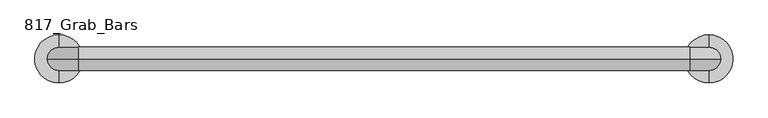
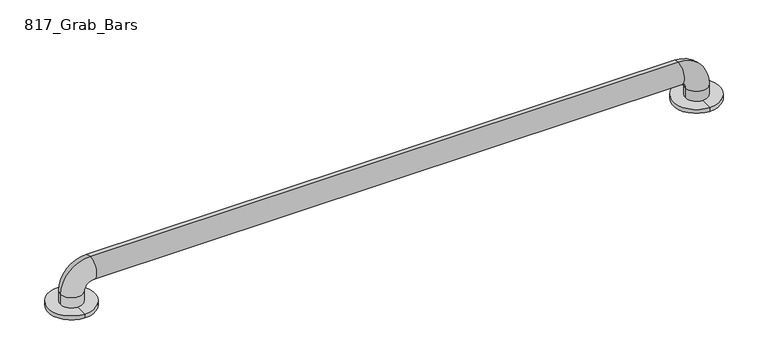
"""IFC4 building model written with IfcOpenShell, lengths in millimetres: proxy geometry, 817_Grab_Bars : 8170-001420."""

from ifc_helpers import new_model, si_unit, point, frame, origin, place, context, project, spatial, circle_curve, ellipse_curve, trimmed, source, transform, mapped, element, save
from ifc_brep_helpers import plane_surface, cylinder_surface, revolved_surface, advanced_brep


def proxy_817_grab_bars_e388bd4b(model_context):
    return source(origin(), model_context, "Body", "AdvancedBrep", [
        advanced_brep(
        [(-439.7375, -496.8875, 7.14375), (-439.7375, -576.2625, 7.14375), (-439.7375, -555.625, 7.14375), (-458.7875, -536.575, 7.14375), (-439.7375, -517.525, 7.14375), (-420.6875, -536.575, 7.14375), (-439.7375, -576.2625, 0.0), (-439.7375, -496.8875, 0.0), (-439.7375, -517.525, 0.0), (-439.7375, -536.575, 0.0), (-439.7375, -555.625, 0.0), (627.0625, -496.8875, 7.14375), (627.0625, -576.2625, 7.14375), (627.0625, -555.625, 7.14375), (608.0125, -536.575, 7.14375), (627.0625, -517.525, 7.14375), (646.1125, -536.575, 7.14375), (627.0625, -576.2625, 0.0), (627.0625, -496.8875, 0.0), (627.0625, -517.525, 0.0), (627.0625, -536.575, 0.0), (627.0625, -555.625, 0.0), (-458.7875, -536.575, 25.4), (-420.6875, -536.575, 25.4), (-407.9875, -536.575, 76.2), (-407.9875, -536.575, 38.1), (595.3125, -536.575, 76.2), (595.3125, -536.575, 38.1), (646.1125, -536.575, 25.4), (608.0125, -536.575, 25.4)],
        [
            (0, 1, circle_curve(frame((-439.7375, -536.575, 7.14375), z_axis=(0.0, 0.0, 1.0), x_axis=(0.0, 1.0, 0.0)), 39.6875)),
            (1, 2),
            (2, 3, circle_curve(frame((-439.7375, -536.575, 7.14375), z_axis=(0.0, 0.0, -1.0), x_axis=(1.0, 0.0, 0.0)), 19.05)),
            (3, 4, circle_curve(frame((-439.7375, -536.575, 7.14375), z_axis=(0.0, 0.0, -1.0), x_axis=(1.0, 0.0, 0.0)), 19.05)),
            (4, 0),
            (1, 0, circle_curve(frame((-439.7375, -536.575, 7.14375), z_axis=(0.0, 0.0, 1.0), x_axis=(0.0, 1.0, 0.0)), 39.6875)),
            (4, 5, circle_curve(frame((-439.7375, -536.575, 7.14375), z_axis=(0.0, 0.0, -1.0), x_axis=(1.0, 0.0, 0.0)), 19.05)),
            (5, 2, circle_curve(frame((-439.7375, -536.575, 7.14375), z_axis=(0.0, 0.0, -1.0), x_axis=(1.0, 0.0, 0.0)), 19.05)),
            (6, 7, circle_curve(frame((-439.7375, -536.575, 0.0), z_axis=(0.0, 0.0, -1.0), x_axis=(0.0, 1.0, 0.0)), 39.6875)),
            (7, 8),
            (8, 9),
            (9, 10),
            (10, 6),
            (7, 6, circle_curve(frame((-439.7375, -536.575, 0.0), z_axis=(0.0, 0.0, -1.0), x_axis=(0.0, 1.0, 0.0)), 39.6875)),
            (0, 7),
            (6, 1),
            (11, 12, circle_curve(frame((627.0625, -536.575, 7.14375), z_axis=(0.0, 0.0, 1.0), x_axis=(0.0, 1.0, 0.0)), 39.6875)),
            (12, 13),
            (13, 14, circle_curve(frame((627.0625, -536.575, 7.14375), z_axis=(0.0, 0.0, -1.0), x_axis=(-1.0, 0.0, 0.0)), 19.05)),
            (14, 15, circle_curve(frame((627.0625, -536.575, 7.14375), z_axis=(0.0, 0.0, -1.0), x_axis=(-1.0, 0.0, 0.0)), 19.05)),
            (15, 11),
            (12, 11, circle_curve(frame((627.0625, -536.575, 7.14375), z_axis=(0.0, 0.0, 1.0), x_axis=(0.0, 1.0, 0.0)), 39.6875)),
            (15, 16, circle_curve(frame((627.0625, -536.575, 7.14375), z_axis=(0.0, 0.0, -1.0), x_axis=(-1.0, 0.0, 0.0)), 19.05)),
            (16, 13, circle_curve(frame((627.0625, -536.575, 7.14375), z_axis=(0.0, 0.0, -1.0), x_axis=(-1.0, 0.0, 0.0)), 19.05)),
            (17, 18, circle_curve(frame((627.0625, -536.575, 0.0), z_axis=(0.0, 0.0, -1.0), x_axis=(0.0, 1.0, 0.0)), 39.6875)),
            (18, 19),
            (19, 20),
            (20, 21),
            (21, 17),
            (18, 17, circle_curve(frame((627.0625, -536.575, 0.0), z_axis=(0.0, 0.0, -1.0), x_axis=(0.0, 1.0, 0.0)), 39.6875)),
            (11, 18),
            (17, 12),
            (22, 23, circle_curve(frame((-439.7375, -536.575, 25.4), z_axis=(0.0, 0.0, -1.0), x_axis=(1.0, 0.0, 0.0)), 19.05)),
            (23, 5),
            (3, 22),
            (23, 22, circle_curve(frame((-439.7375, -536.575, 25.4), z_axis=(0.0, 0.0, -1.0), x_axis=(1.0, 0.0, 0.0)), 19.05)),
            (22, 24, circle_curve(frame((-407.9875, -536.575, 25.4), z_axis=(0.0, 1.0, 0.0), x_axis=(-1.0, 0.0, 0.0)), 50.8)),
            (24, 25, circle_curve(frame((-407.9875, -536.575, 57.15), z_axis=(-1.0, 0.0, 0.0), x_axis=(0.0, 0.0, -1.0)), 19.05)),
            (25, 23, circle_curve(frame((-407.9875, -536.575, 25.4), z_axis=(0.0, -1.0, 0.0), x_axis=(-1.0, 0.0, 0.0)), 12.7)),
            (25, 24, circle_curve(frame((-407.9875, -536.575, 57.15), z_axis=(-1.0, 0.0, 0.0), x_axis=(0.0, 0.0, -1.0)), 19.05)),
            (24, 26),
            (26, 27, circle_curve(frame((595.3125, -536.575, 57.15), z_axis=(-1.0, 0.0, 0.0), x_axis=(0.0, 0.0, -1.0)), 19.05)),
            (27, 25),
            (27, 26, circle_curve(frame((595.3125, -536.575, 57.15), z_axis=(-1.0, 0.0, 0.0), x_axis=(0.0, 0.0, -1.0)), 19.05)),
            (26, 28, circle_curve(frame((595.3125, -536.575, 25.4), z_axis=(0.0, 1.0, 0.0), x_axis=(0.0, 0.0, 1.0)), 50.8)),
            (28, 29, circle_curve(frame((627.0625, -536.575, 25.4), z_axis=(0.0, 0.0, 1.0), x_axis=(-1.0, 0.0, 0.0)), 19.05)),
            (29, 27, circle_curve(frame((595.3125, -536.575, 25.4), z_axis=(0.0, -1.0, 0.0), x_axis=(0.0, 0.0, 1.0)), 12.7)),
            (29, 28, circle_curve(frame((627.0625, -536.575, 25.4), z_axis=(0.0, 0.0, 1.0), x_axis=(-1.0, 0.0, 0.0)), 19.05)),
            (28, 16),
            (14, 29),
        ],
        [
            plane_surface(frame((-439.7375, -536.575, 7.14375), z_axis=(0.0, 0.0, 1.0), x_axis=(0.0, 1.0, 0.0))),
            plane_surface(frame((-439.7375, -536.575, 0.0), z_axis=(0.0, 0.0, -1.0), x_axis=(0.0, 1.0, 0.0))),
            cylinder_surface(frame((-439.7375, -536.575, 7.14375), z_axis=(0.0, 0.0, 1.0), x_axis=(0.0, 1.0, 0.0)), 39.6875),
            plane_surface(frame((627.0625, -536.575, 7.14375), z_axis=(0.0, 0.0, 1.0), x_axis=(0.0, 1.0, 0.0))),
            plane_surface(frame((627.0625, -536.575, 0.0), z_axis=(0.0, 0.0, -1.0), x_axis=(0.0, 1.0, 0.0))),
            cylinder_surface(frame((627.0625, -536.575, 31.75), z_axis=(0.0, 0.0, 1.0), x_axis=(0.0, 1.0, 0.0)), 39.6875),
            cylinder_surface(frame((-439.7375, -536.575, 0.0), z_axis=(0.0, 0.0, -1.0), x_axis=(1.0, 0.0, 0.0)), 19.05),
            revolved_surface(trimmed(ellipse_curve(frame((-439.7375, -536.575, 25.4), z_axis=(0.0, 0.0, -1.0), x_axis=(1.0, 0.0, 0.0)), 19.05, 19.05), [point((-458.7875, -536.575, 25.4))], [point((-420.6875, -536.575, 25.4))], True, "CARTESIAN"), (-407.9875, -536.575, 25.4), (0.0, 1.0, 0.0)),
            revolved_surface(trimmed(ellipse_curve(frame((-439.7375, -536.575, 25.4), z_axis=(0.0, 0.0, -1.0), x_axis=(1.0, 0.0, 0.0)), 19.05, 19.05), [point((-420.6875, -536.575, 25.4))], [point((-458.7875, -536.575, 25.4))], True, "CARTESIAN"), (-407.9875, -536.575, 25.4), (0.0, 1.0, 0.0)),
            cylinder_surface(frame((-407.9875, -536.575, 57.15), z_axis=(-1.0, 0.0, 0.0), x_axis=(0.0, 0.0, -1.0)), 19.05),
            revolved_surface(trimmed(ellipse_curve(frame((595.3125, -536.575, 57.15), z_axis=(-1.0, 0.0, 0.0), x_axis=(0.0, 0.0, -1.0)), 19.05, 19.05), [point((595.3125, -536.575, 76.2))], [point((595.3125, -536.575, 38.1))], True, "CARTESIAN"), (595.3125, -536.575, 25.4), (0.0, 1.0, 0.0)),
            revolved_surface(trimmed(ellipse_curve(frame((595.3125, -536.575, 57.15), z_axis=(-1.0, 0.0, 0.0), x_axis=(0.0, 0.0, -1.0)), 19.05, 19.05), [point((595.3125, -536.575, 38.1))], [point((595.3125, -536.575, 76.2))], True, "CARTESIAN"), (595.3125, -536.575, 25.4), (0.0, 1.0, 0.0)),
            cylinder_surface(frame((627.0625, -536.575, 25.4), z_axis=(0.0, 0.0, 1.0), x_axis=(-1.0, 0.0, 0.0)), 19.05),
        ],
        [
            (0, [[1, 2, 3, 4, 5]]),
            (0, [[6, -5, 7, 8, -2]]),
            (1, [[9, 10, 11, 12, 13]]),
            (1, [[14, -13, -12, -11, -10]]),
            (2, [[-1, 15, -9, 16]]),
            (2, [[-6, -16, -14, -15]]),
            (3, [[17, 18, 19, 20, 21]]),
            (3, [[22, -21, 23, 24, -18]]),
            (4, [[25, 26, 27, 28, 29]]),
            (4, [[30, -29, -28, -27, -26]]),
            (5, [[-17, 31, -25, 32]]),
            (5, [[-22, -32, -30, -31]]),
            (6, [[33, 34, -7, -4, 35]]),
            (6, [[36, -35, -3, -8, -34]]),
            (7, [[-33, 37, 38, 39]]),
            (8, [[-36, -39, 40, -37]]),
            (9, [[-38, 41, 42, 43]]),
            (9, [[-40, -43, 44, -41]]),
            (10, [[-42, 45, 46, 47]]),
            (11, [[-44, -47, 48, -45]]),
            (12, [[-46, 49, -23, -20, 50]]),
            (12, [[-48, -50, -19, -24, -49]]),
        ],
    ),
    ])


if __name__ == "__main__":
    model = new_model("IFC4")
    model_context = context("Model", 3, world=origin())
    ifc_project = project(units=[si_unit("LENGTHUNIT", "METRE", prefix="MILLI")], contexts=[model_context])
    site = spatial("IfcSite", under=ifc_project)
    building = spatial("IfcBuilding", under=site)
    placement = place(None, origin())
    proxy_817_grab_bars_shape = proxy_817_grab_bars_e388bd4b(model_context)
    element("IfcBuildingElementProxy", 1, Name="817_Grab_Bars : 8170-001420", ObjectType="817_Grab_Bars : 8170-001420", at=placement, inside=building, context=model_context, shape_type="MappedRepresentation", body=[
        mapped(proxy_817_grab_bars_shape, transform((0.0, 0.0, 0.0), x_axis=(1.0, 0.0, 0.0), y_axis=(0.0, 1.0, 0.0), z_axis=(0.0, 0.0, 1.0))),
    ])
    save(model, "model.ifc")

# Revit data of these elements
# Type "817_Grab_Bars : 8170-001420"
#   Keynote = "M10281313.01"
#   Warranty Information = "Complete unit, one (1) year"
#   Version = "1.0"
#   Technical Data = "http://www.bradleycorp.com/products/techdata/8815.pdf"
#   URL = "www.bradleycorp.com"
#   Type Comments = "All grab bar configurations are specified using centerline to centerline dimensions."
#   OmniClass Title = ""
#   Modeling Code = ""
#   Model = "8170-001420"
#   Material Note = "FLANGES - 11 GA., TUBING - 18 GA."
#   MasterFormat Section Title = ""
#   Manufacturer = "Bradley Corporation"
#   LEED Credit = ""
#   Instructions [instance default] = "This is a face mounted fixture."
#   Industry Standards = "ANSI Standard A117.1, ADA, ABA, ADAAG, UFAS"
#   Fire Rating = "None"
#   Description = "Grab Bars"
#   Copyright = "This Model Data is Property of Bradley Corporation"
#   Complies to NAFTA = "Yes"
#   Complies To Buy American Act = "Yes"
#   Assembly Code = "C1030200"
#   ADA Compliant = "Yes"
#   Radius = 0' - 0 3/4"
#   Percentage of Recycled Content = 56.77
#   Overall Length = 3' - 9 1/8"
#   OmniClass Number = 0
#   MasterFormat Section Number = 0
#   Length = 3' - 6"
#   Diameter = 0' - 1 1/2"
#   Default Elevation = 2' - 9"
#   Material and Finish = Bradley Corp Stainless Steel - Satin
# Element 1 (IfcBuildingElementProxy, "817_Grab_Bars : 8170-001420")
#   Materials on its faces: "Bradley Corp Stainless Steel - Satin"
# Materials
#   "Bradley Corp Stainless Steel - Satin": class "Metal", colour RGB 189 187 185, transparency 0, Manufacturer = "Bradley Corporation", URL = "www.bradleycorp.com", Description = "Stainless Steel - Satin Finish", Cost = 0
